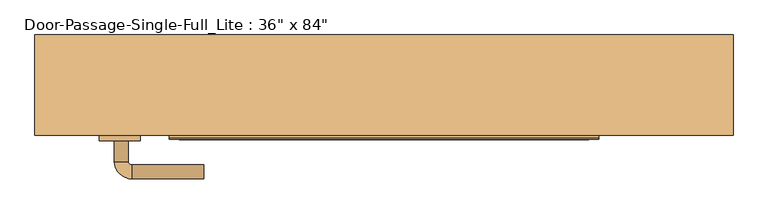
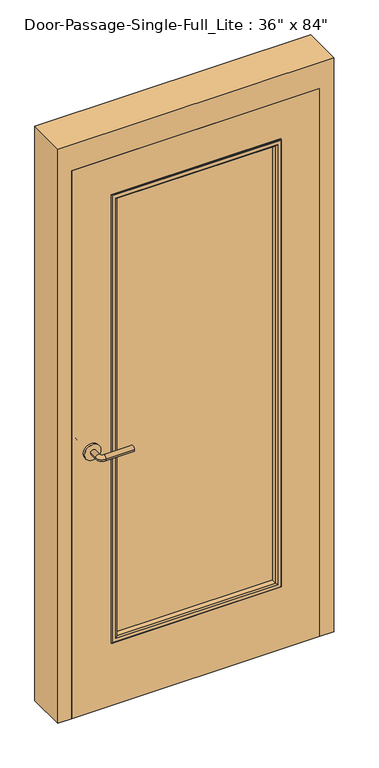
"""IFC4 building model written with IfcOpenShell, lengths in millimetres: door geometry."""

from ifc_helpers import new_model, si_unit, point, frame, frame_2d, origin, place, context, project, spatial, polyline, circle_curve, ellipse_curve, trimmed, segment, composite_curve, outline, extrude, faceted_brep, source, transform, mapped, element, save
from ifc_brep_helpers import plane_surface, cylinder_surface, revolved_surface, advanced_brep


def door_5fc50167(model_context):
    return source(origin(), model_context, "Body", "SolidModel", [
        advanced_brep(
        [(-392.190625, 9.5875, 1016.0), (-372.190625, 9.5875, 1016.0), (-392.190625, 39.5875, 1016.0), (-372.190625, 39.5875, 1016.0), (-367.190625, 44.5875, 1016.0), (-367.190625, 64.5875, 1016.0), (-262.190625, 64.5875, 1016.0), (-262.190625, 44.5875, 1016.0)],
        [
            (0, 1, circle_curve(frame((-382.190625, 9.5875, 1016.0), z_axis=(0.0, -1.0, 0.0), x_axis=(1.0, 0.0, 0.0)), 10.0)),
            (1, 0, circle_curve(frame((-382.190625, 9.5875, 1016.0), z_axis=(0.0, -1.0, 0.0), x_axis=(1.0, 0.0, 0.0)), 10.0)),
            (0, 2),
            (2, 3, circle_curve(frame((-382.190625, 39.5875, 1016.0), z_axis=(0.0, -1.0, 0.0), x_axis=(1.0, 0.0, 0.0)), 10.0)),
            (3, 1),
            (3, 2, circle_curve(frame((-382.190625, 39.5875, 1016.0), z_axis=(0.0, -1.0, 0.0), x_axis=(1.0, 0.0, 0.0)), 10.0)),
            (4, 3, circle_curve(frame((-367.190625, 39.5875, 1016.0), z_axis=(0.0, 0.0, 1.0), x_axis=(-1.0, 0.0, 0.0)), 5.0)),
            (2, 5, circle_curve(frame((-367.190625, 39.5875, 1016.0), z_axis=(0.0, 0.0, -1.0), x_axis=(-1.0, 0.0, 0.0)), 25.0)),
            (5, 4, circle_curve(frame((-367.190625, 54.5875, 1016.0), z_axis=(-1.0, 0.0, 0.0), x_axis=(0.0, -1.0, 0.0)), 10.0)),
            (4, 5, circle_curve(frame((-367.190625, 54.5875, 1016.0), z_axis=(-1.0, 0.0, 0.0), x_axis=(0.0, -1.0, 0.0)), 10.0)),
            (6, 7, circle_curve(frame((-262.190625, 54.5875, 1016.0), z_axis=(1.0, 0.0, 0.0), x_axis=(0.0, -1.0, 0.0)), 10.0)),
            (7, 6, circle_curve(frame((-262.190625, 54.5875, 1016.0), z_axis=(1.0, 0.0, 0.0), x_axis=(0.0, -1.0, 0.0)), 10.0)),
            (5, 6),
            (7, 4),
        ],
        [
            plane_surface(frame((-382.190625, 9.5875, 1016.0), z_axis=(0.0, -1.0, 0.0), x_axis=(0.0, 0.0, 1.0))),
            cylinder_surface(frame((-382.190625, 9.5875, 1016.0), z_axis=(0.0, -1.0, 0.0), x_axis=(1.0, 0.0, 0.0)), 10.0),
            revolved_surface(trimmed(ellipse_curve(frame((-382.190625, 39.5875, 1016.0), z_axis=(0.0, -1.0, 0.0), x_axis=(1.0, 0.0, 0.0)), 10.0, 10.0), [point((-392.190625, 39.5875, 1016.0))], [point((-372.190625, 39.5875, 1016.0))], True, "CARTESIAN"), (-367.190625, 39.5875, 1016.0), (0.0, 0.0, -1.0)),
            revolved_surface(trimmed(ellipse_curve(frame((-382.190625, 39.5875, 1016.0), z_axis=(0.0, -1.0, 0.0), x_axis=(1.0, 0.0, 0.0)), 10.0, 10.0), [point((-372.190625, 39.5875, 1016.0))], [point((-392.190625, 39.5875, 1016.0))], True, "CARTESIAN"), (-367.190625, 39.5875, 1016.0), (0.0, 0.0, -1.0)),
            plane_surface(frame((-262.190625, 54.5875, 1016.0), z_axis=(1.0, 0.0, 0.0), x_axis=(0.0, 0.0, 1.0))),
            cylinder_surface(frame((-367.190625, 54.5875, 1016.0), z_axis=(-1.0, 0.0, 0.0), x_axis=(0.0, -1.0, 0.0)), 10.0),
        ],
        [
            (0, [[1, 2]]),
            (1, [[-1, 3, 4, 5]]),
            (1, [[-2, -5, 6, -3]]),
            (2, [[7, -4, 8, 9]]),
            (3, [[-8, -6, -7, 10]]),
            (4, [[11, 12]]),
            (5, [[-9, 13, -12, 14]]),
            (5, [[-10, -14, -11, -13]]),
        ],
    ),
        extrude(outline(composite_curve([segment(trimmed(circle_curve(frame_2d((1016.0, -384.690625)), 30.0), [point((1016.0, -414.690625))], [point((1016.0, -354.690625))], False, "CARTESIAN"), True, "CONTINUOUS"), segment(trimmed(circle_curve(frame_2d((1016.0, -384.690625)), 30.0), [point((1016.0, -354.690625))], [point((1016.0, -414.690625))], False, "CARTESIAN"), True, "CONTINUOUS")], self_intersect=False)), frame((0.0, 1.5875, 0.0), z_axis=(0.0, 1.0, 0.0), x_axis=(0.0, 0.0, 1.0)), (0.0, 0.0, 1.0), 8.0),
        advanced_brep(
        [(-392.190625, -50.8625, 1016.0), (-372.190625, -50.8625, 1016.0), (-372.190625, -80.8625, 1016.0), (-392.190625, -80.8625, 1016.0), (-367.190625, -85.8625, 1016.0), (-367.190625, -105.8625, 1016.0), (-262.190625, -105.8625, 1016.0), (-262.190625, -85.8625, 1016.0)],
        [
            (0, 1, circle_curve(frame((-382.190625, -50.8625, 1016.0), z_axis=(0.0, 1.0, 0.0), x_axis=(1.0, 0.0, 0.0)), 10.0)),
            (1, 0, circle_curve(frame((-382.190625, -50.8625, 1016.0), z_axis=(0.0, 1.0, 0.0), x_axis=(1.0, 0.0, 0.0)), 10.0)),
            (1, 2),
            (2, 3, circle_curve(frame((-382.190625, -80.8625, 1016.0), z_axis=(0.0, 1.0, 0.0), x_axis=(1.0, 0.0, 0.0)), 10.0)),
            (3, 0),
            (3, 2, circle_curve(frame((-382.190625, -80.8625, 1016.0), z_axis=(0.0, 1.0, 0.0), x_axis=(1.0, 0.0, 0.0)), 10.0)),
            (4, 5, circle_curve(frame((-367.190625, -95.8625, 1016.0), z_axis=(-1.0, 0.0, 0.0), x_axis=(0.0, 1.0, 0.0)), 10.0)),
            (5, 3, circle_curve(frame((-367.190625, -80.8625, 1016.0), z_axis=(0.0, 0.0, -1.0), x_axis=(-1.0, 0.0, 0.0)), 25.0)),
            (2, 4, circle_curve(frame((-367.190625, -80.8625, 1016.0), z_axis=(0.0, 0.0, 1.0), x_axis=(-1.0, 0.0, 0.0)), 5.0)),
            (5, 4, circle_curve(frame((-367.190625, -95.8625, 1016.0), z_axis=(-1.0, 0.0, 0.0), x_axis=(0.0, 1.0, 0.0)), 10.0)),
            (6, 7, circle_curve(frame((-262.190625, -95.8625, 1016.0), z_axis=(1.0, 0.0, 0.0), x_axis=(0.0, 1.0, 0.0)), 10.0)),
            (7, 6, circle_curve(frame((-262.190625, -95.8625, 1016.0), z_axis=(1.0, 0.0, 0.0), x_axis=(0.0, 1.0, 0.0)), 10.0)),
            (4, 7),
            (6, 5),
        ],
        [
            plane_surface(frame((-382.190625, -50.8625, 1016.0), z_axis=(0.0, 1.0, 0.0), x_axis=(0.0, 0.0, 1.0))),
            cylinder_surface(frame((-382.190625, -50.8625, 1016.0), z_axis=(0.0, 1.0, 0.0), x_axis=(1.0, 0.0, 0.0)), 10.0),
            revolved_surface(trimmed(ellipse_curve(frame((-382.190625, -80.8625, 1016.0), z_axis=(0.0, -1.0, 0.0), x_axis=(1.0, 0.0, 0.0)), 10.0, 10.0), [point((-392.190625, -80.8625, 1016.0))], [point((-372.190625, -80.8625, 1016.0))], True, "CARTESIAN"), (-367.190625, -80.8625, 1016.0), (0.0, 0.0, -1.0)),
            revolved_surface(trimmed(ellipse_curve(frame((-382.190625, -80.8625, 1016.0), z_axis=(0.0, -1.0, 0.0), x_axis=(1.0, 0.0, 0.0)), 10.0, 10.0), [point((-372.190625, -80.8625, 1016.0))], [point((-392.190625, -80.8625, 1016.0))], True, "CARTESIAN"), (-367.190625, -80.8625, 1016.0), (0.0, 0.0, -1.0)),
            plane_surface(frame((-262.190625, -95.8625, 1016.0), z_axis=(1.0, 0.0, 0.0), x_axis=(0.0, 0.0, 1.0))),
            cylinder_surface(frame((-367.190625, -95.8625, 1016.0), z_axis=(-1.0, 0.0, 0.0), x_axis=(0.0, 1.0, 0.0)), 10.0),
        ],
        [
            (0, [[1, 2]]),
            (1, [[3, 4, 5, -2]]),
            (1, [[-5, 6, -3, -1]]),
            (2, [[7, 8, -4, 9]]),
            (3, [[10, -9, -6, -8]]),
            (4, [[11, 12]]),
            (5, [[13, -11, 14, -7]]),
            (5, [[-14, -12, -13, -10]]),
        ],
    ),
        extrude(outline(composite_curve([segment(trimmed(circle_curve(frame_2d((1016.0, -384.690625)), 30.0), [point((1016.0, -414.690625))], [point((1016.0, -354.690625))], False, "CARTESIAN"), True, "CONTINUOUS"), segment(trimmed(circle_curve(frame_2d((1016.0, -384.690625)), 30.0), [point((1016.0, -354.690625))], [point((1016.0, -414.690625))], False, "CARTESIAN"), True, "CONTINUOUS")], self_intersect=False)), frame((0.0, -50.8625, 0.0), z_axis=(0.0, 1.0, 0.0), x_axis=(0.0, 0.0, 1.0)), (0.0, 0.0, 1.0), 8.0),
        extrude(outline(polyline([(304.8, -17.4625), (304.8, -23.8125), (-304.8, -23.8125), (-304.8, -17.4625), (304.8, -17.4625)])), frame((0.0, 0.0, 254.0), z_axis=(0.0, 0.0, 1.0), x_axis=(1.0, 0.0, 0.0)), (0.0, 0.0, 1.0), 1727.2),
        faceted_brep([(457.2, 6.35, 0.0), (441.325, 6.35, 0.0), (441.325, 53.975, 0.0), (457.2, 53.975, 0.0), (457.2, 103.1875, 0.0), (508.0, 103.1875, 0.0), (508.0, -42.8625, 0.0), (457.2, -42.8625, 0.0), (457.2, -42.8625, 2133.6), (457.2, 6.35, 2133.6), (508.0, -42.8625, 2235.2), (-508.0, -42.8625, 2235.2), (-508.0, -42.8625, 0.0), (-457.2, -42.8625, 0.0), (-457.2, -42.8625, 2133.6), (508.0, 103.1875, 2235.2), (457.2, 103.1875, 2133.6), (-457.2, 103.1875, 2133.6), (-457.2, 103.1875, 0.0), (-508.0, 103.1875, 0.0), (-508.0, 103.1875, 2235.2), (457.2, 53.975, 2133.6), (441.325, 53.975, 2117.725), (-441.325, 53.975, 2117.725), (-441.325, 53.975, 0.0), (-457.2, 53.975, 0.0), (-457.2, 53.975, 2133.6), (441.325, 6.35, 2117.725), (-457.2, 6.35, 2133.6), (-457.2, 6.35, 0.0), (-441.325, 6.35, 0.0), (-441.325, 6.35, 2117.725)], [[[0, 1, 2, 3, 4, 5, 6, 7]], [[7, 8, 9, 0]], [[6, 10, 11, 12, 13, 14, 8, 7]], [[5, 15, 10, 6]], [[4, 16, 17, 18, 19, 20, 15, 5]], [[3, 21, 16, 4]], [[2, 22, 23, 24, 25, 26, 21, 3]], [[1, 27, 22, 2]], [[0, 9, 28, 29, 30, 31, 27, 1]], [[8, 14, 28, 9]], [[16, 21, 26, 17]], [[22, 27, 31, 23]], [[12, 19, 18, 25, 24, 30, 29, 13]], [[13, 29, 28, 14]], [[11, 20, 19, 12]], [[17, 26, 25, 18]], [[23, 31, 30, 24]], [[15, 20, 11, 10]]]),
        extrude(outline(polyline([(2133.6, -457.2), (0.0, -457.2), (0.0, 457.2), (2133.6, 457.2), (2133.6, -457.2)]), holes=[polyline([(1981.2, -304.8), (1981.2, 304.8), (254.0, 304.8), (254.0, -304.8), (1981.2, -304.8)])]), frame((0.0, -42.8625, 0.0), z_axis=(0.0, 1.0, 0.0), x_axis=(0.0, 0.0, 1.0)), (0.0, 0.0, 1.0), 44.45),
        advanced_brep(
        [(-304.8, -23.8125, 1981.2), (-304.8, -23.8125, 254.0), (-304.8, -42.8625, 254.0), (-304.8, -42.8625, 1981.2), (-292.8, -43.8625, 1969.2), (-292.8, -43.8625, 266.0), (-292.8, -23.8125, 266.0), (-292.8, -23.8125, 1969.2), (-297.8, -48.8625, 1974.2), (-297.8, -48.8625, 261.0), (-312.8, -46.8625, 1989.2), (-312.8, -46.8625, 246.0), (-310.8, -48.8625, 248.0), (-310.8, -48.8625, 1987.2), (-312.8, -42.8625, 1989.2), (-312.8, -42.8625, 246.0), (304.8, -23.8125, 254.0), (304.8, -42.8625, 254.0), (292.8, -43.8625, 266.0), (292.8, -23.8125, 266.0), (297.8, -48.8625, 261.0), (312.8, -46.8625, 246.0), (310.8, -48.8625, 248.0), (312.8, -42.8625, 246.0), (304.8, -23.8125, 1981.2), (304.8, -42.8625, 1981.2), (292.8, -43.8625, 1969.2), (292.8, -23.8125, 1969.2), (297.8, -48.8625, 1974.2), (312.8, -46.8625, 1989.2), (310.8, -48.8625, 1987.2), (312.8, -42.8625, 1989.2)],
        [
            (0, 1),
            (1, 2),
            (2, 3),
            (3, 0),
            (4, 5),
            (5, 6),
            (6, 7),
            (7, 4),
            (8, 9),
            (9, 5, ellipse_curve(frame((-297.8, -43.8625, 261.0), z_axis=(-0.7071067811865475, 0.0, 0.7071067811865475), x_axis=(0.7071067811865474, 0.0, 0.7071067811865476)), 7.0710678, 5.0)),
            (4, 8, ellipse_curve(frame((-297.8, -43.8625, 1974.2), z_axis=(-0.7071067811865475, 0.0, -0.7071067811865475), x_axis=(-0.7071067811865474, 0.0, 0.7071067811865476)), 7.0710678, 5.0)),
            (10, 11),
            (11, 12, ellipse_curve(frame((-310.8, -46.8625, 248.0), z_axis=(-0.7071067811865475, 0.0, 0.7071067811865475), x_axis=(0.7071067811865474, 0.0, 0.7071067811865476)), 2.8284271, 2.0)),
            (12, 13),
            (13, 10, ellipse_curve(frame((-310.8, -46.8625, 1987.2), z_axis=(-0.7071067811865475, 0.0, -0.7071067811865475), x_axis=(-0.7071067811865474, 0.0, 0.7071067811865476)), 2.8284271, 2.0)),
            (14, 15),
            (15, 11),
            (10, 14),
            (1, 16),
            (16, 17),
            (17, 2),
            (5, 18),
            (18, 19),
            (19, 6),
            (9, 20),
            (20, 18, ellipse_curve(frame((297.8, -43.8625, 261.0), z_axis=(-0.7071067811865475, 0.0, -0.7071067811865475), x_axis=(-0.7071067811865476, 0.0, 0.7071067811865474)), 7.0710678, 5.0)),
            (11, 21),
            (21, 22, ellipse_curve(frame((310.8, -46.8625, 248.0), z_axis=(-0.7071067811865475, 0.0, -0.7071067811865475), x_axis=(-0.7071067811865476, 0.0, 0.7071067811865474)), 2.8284271, 2.0)),
            (22, 12),
            (15, 23),
            (23, 21),
            (16, 24),
            (24, 25),
            (25, 17),
            (18, 26),
            (26, 27),
            (27, 19),
            (20, 28),
            (28, 26, ellipse_curve(frame((297.8, -43.8625, 1974.2), z_axis=(0.7071067811865475, 0.0, -0.7071067811865475), x_axis=(-0.7071067811865474, 0.0, -0.7071067811865476)), 7.0710678, 5.0)),
            (21, 29),
            (29, 30, ellipse_curve(frame((310.8, -46.8625, 1987.2), z_axis=(0.7071067811865475, 0.0, -0.7071067811865475), x_axis=(-0.7071067811865474, 0.0, -0.7071067811865476)), 2.8284271, 2.0)),
            (30, 22),
            (23, 31),
            (31, 29),
            (14, 31),
            (25, 3),
            (24, 0),
            (27, 7),
            (26, 4),
            (28, 8),
            (30, 13),
            (29, 10),
        ],
        [
            plane_surface(frame((-304.8, -42.8625, 1981.2), z_axis=(-1.0, 0.0, 0.0), x_axis=(0.0, 0.0, -1.0))),
            plane_surface(frame((-292.8, -23.8125, 1969.2), z_axis=(1.0, 0.0, 0.0), x_axis=(0.0, 0.0, -1.0))),
            cylinder_surface(frame((-297.8, -43.8625, 1981.2), z_axis=(0.0, 0.0, 1.0), x_axis=(-1.0, 0.0, 0.0)), 5.0),
            cylinder_surface(frame((-310.8, -46.8625, 1981.2), z_axis=(0.0, 0.0, 1.0), x_axis=(-1.0, 0.0, 0.0)), 2.0),
            plane_surface(frame((-312.8, -46.8625, 1989.2), z_axis=(-1.0, 0.0, 0.0), x_axis=(0.0, 0.0, -1.0))),
            plane_surface(frame((-304.8, -42.8625, 254.0), z_axis=(0.0, 0.0, -1.0), x_axis=(1.0, 0.0, 0.0))),
            plane_surface(frame((-292.8, -23.8125, 266.0), z_axis=(0.0, 0.0, 1.0), x_axis=(1.0, 0.0, 0.0))),
            cylinder_surface(frame((-304.8, -43.8625, 261.0), z_axis=(-1.0, 0.0, 0.0), x_axis=(0.0, 0.0, -1.0)), 5.0),
            cylinder_surface(frame((-304.8, -46.8625, 248.0), z_axis=(-1.0, 0.0, 0.0), x_axis=(0.0, 0.0, -1.0)), 2.0),
            plane_surface(frame((-312.8, -46.8625, 246.0), z_axis=(0.0, 0.0, -1.0), x_axis=(1.0, 0.0, 0.0))),
            plane_surface(frame((304.8, -42.8625, 254.0), z_axis=(1.0, 0.0, 0.0), x_axis=(0.0, 0.0, 1.0))),
            plane_surface(frame((292.8, -23.8125, 266.0), z_axis=(-1.0, 0.0, 0.0), x_axis=(0.0, 0.0, 1.0))),
            cylinder_surface(frame((297.8, -43.8625, 254.0), z_axis=(0.0, 0.0, -1.0), x_axis=(1.0, 0.0, 0.0)), 5.0),
            cylinder_surface(frame((310.8, -46.8625, 254.0), z_axis=(0.0, 0.0, -1.0), x_axis=(1.0, 0.0, 0.0)), 2.0),
            plane_surface(frame((312.8, -46.8625, 246.0), z_axis=(1.0, 0.0, 0.0), x_axis=(0.0, 0.0, 1.0))),
            plane_surface(frame((312.8, -42.8625, 1989.2), z_axis=(0.0, 1.0, 0.0), x_axis=(-1.0, 0.0, 0.0))),
            plane_surface(frame((304.8, -42.8625, 1981.2), z_axis=(0.0, 0.0, 1.0), x_axis=(-1.0, 0.0, 0.0))),
            plane_surface(frame((304.8, -23.8125, 1981.2), z_axis=(0.0, 1.0, 0.0), x_axis=(-1.0, 0.0, 0.0))),
            plane_surface(frame((292.8, -23.8125, 1969.2), z_axis=(0.0, 0.0, -1.0), x_axis=(-1.0, 0.0, 0.0))),
            cylinder_surface(frame((304.8, -43.8625, 1974.2), z_axis=(1.0, 0.0, 0.0), x_axis=(0.0, 0.0, 1.0)), 5.0),
            plane_surface(frame((297.8, -48.8625, 1974.2), z_axis=(0.0, -1.0, 0.0), x_axis=(-1.0, 0.0, 0.0))),
            cylinder_surface(frame((304.8, -46.8625, 1987.2), z_axis=(1.0, 0.0, 0.0), x_axis=(0.0, 0.0, 1.0)), 2.0),
            plane_surface(frame((312.8, -46.8625, 1989.2), z_axis=(0.0, 0.0, 1.0), x_axis=(-1.0, 0.0, 0.0))),
        ],
        [
            (0, [[1, 2, 3, 4]]),
            (1, [[5, 6, 7, 8]]),
            (2, [[9, 10, -5, 11]]),
            (3, [[12, 13, 14, 15]]),
            (4, [[16, 17, -12, 18]]),
            (5, [[19, 20, 21, -2]]),
            (6, [[22, 23, 24, -6]]),
            (7, [[25, 26, -22, -10]]),
            (8, [[27, 28, 29, -13]]),
            (9, [[30, 31, -27, -17]]),
            (10, [[32, 33, 34, -20]]),
            (11, [[35, 36, 37, -23]]),
            (12, [[38, 39, -35, -26]]),
            (13, [[40, 41, 42, -28]]),
            (14, [[43, 44, -40, -31]]),
            (15, [[-16, 45, -43, -30], [-3, -21, -34, 46]]),
            (16, [[47, -4, -46, -33]]),
            (17, [[-1, -47, -32, -19], [-7, -24, -37, 48]]),
            (18, [[49, -8, -48, -36]]),
            (19, [[50, -11, -49, -39]]),
            (20, [[-14, -29, -42, 51], [-9, -50, -38, -25]]),
            (21, [[52, -15, -51, -41]]),
            (22, [[-45, -18, -52, -44]]),
        ],
    ),
        advanced_brep(
        [(-304.8, -17.4625, 254.0), (-304.8, -17.4625, 1981.2), (-304.8, 1.5875, 1981.2), (-304.8, 1.5875, 254.0), (-292.8, 2.5875, 266.0), (-292.8, 2.5875, 1969.2), (-292.8, -17.4625, 1969.2), (-292.8, -17.4625, 266.0), (-297.8, 7.5875, 261.0), (-297.8, 7.5875, 1974.2), (-312.8, 5.5875, 246.0), (-312.8, 5.5875, 1989.2), (-310.8, 7.5875, 1987.2), (-310.8, 7.5875, 248.0), (-312.8, 1.5875, 246.0), (-312.8, 1.5875, 1989.2), (304.8, -17.4625, 1981.2), (304.8, 1.5875, 1981.2), (292.8, 2.5875, 1969.2), (292.8, -17.4625, 1969.2), (297.8, 7.5875, 1974.2), (312.8, 5.5875, 1989.2), (310.8, 7.5875, 1987.2), (312.8, 1.5875, 1989.2), (304.8, -17.4625, 254.0), (304.8, 1.5875, 254.0), (292.8, 2.5875, 266.0), (292.8, -17.4625, 266.0), (297.8, 7.5875, 261.0), (312.8, 5.5875, 246.0), (310.8, 7.5875, 248.0), (312.8, 1.5875, 246.0)],
        [
            (0, 1),
            (1, 2),
            (2, 3),
            (3, 0),
            (4, 5),
            (5, 6),
            (6, 7),
            (7, 4),
            (8, 9),
            (9, 5, ellipse_curve(frame((-297.8, 2.5875, 1974.2), z_axis=(-0.7071067811865475, 0.0, -0.7071067811865475), x_axis=(0.7071067811865474, 0.0, -0.7071067811865476)), 7.0710678, 5.0)),
            (4, 8, ellipse_curve(frame((-297.8, 2.5875, 261.0), z_axis=(-0.7071067811865475, 0.0, 0.7071067811865475), x_axis=(-0.7071067811865474, 0.0, -0.7071067811865476)), 7.0710678, 5.0)),
            (10, 11),
            (11, 12, ellipse_curve(frame((-310.8, 5.5875, 1987.2), z_axis=(-0.7071067811865475, 0.0, -0.7071067811865475), x_axis=(0.7071067811865474, 0.0, -0.7071067811865476)), 2.8284271, 2.0)),
            (12, 13),
            (13, 10, ellipse_curve(frame((-310.8, 5.5875, 248.0), z_axis=(-0.7071067811865475, 0.0, 0.7071067811865475), x_axis=(-0.7071067811865474, 0.0, -0.7071067811865476)), 2.8284271, 2.0)),
            (14, 15),
            (15, 11),
            (10, 14),
            (1, 16),
            (16, 17),
            (17, 2),
            (5, 18),
            (18, 19),
            (19, 6),
            (9, 20),
            (20, 18, ellipse_curve(frame((297.8, 2.5875, 1974.2), z_axis=(-0.7071067811865475, 0.0, 0.7071067811865475), x_axis=(-0.7071067811865476, 0.0, -0.7071067811865474)), 7.0710678, 5.0)),
            (11, 21),
            (21, 22, ellipse_curve(frame((310.8, 5.5875, 1987.2), z_axis=(-0.7071067811865475, 0.0, 0.7071067811865475), x_axis=(-0.7071067811865476, 0.0, -0.7071067811865474)), 2.8284271, 2.0)),
            (22, 12),
            (15, 23),
            (23, 21),
            (16, 24),
            (24, 25),
            (25, 17),
            (18, 26),
            (26, 27),
            (27, 19),
            (20, 28),
            (28, 26, ellipse_curve(frame((297.8, 2.5875, 261.0), z_axis=(0.7071067811865475, 0.0, 0.7071067811865475), x_axis=(-0.7071067811865474, 0.0, 0.7071067811865476)), 7.0710678, 5.0)),
            (21, 29),
            (29, 30, ellipse_curve(frame((310.8, 5.5875, 248.0), z_axis=(0.7071067811865475, 0.0, 0.7071067811865475), x_axis=(-0.7071067811865474, 0.0, 0.7071067811865476)), 2.8284271, 2.0)),
            (30, 22),
            (23, 31),
            (31, 29),
            (14, 31),
            (25, 3),
            (24, 0),
            (27, 7),
            (26, 4),
            (28, 8),
            (30, 13),
            (29, 10),
        ],
        [
            plane_surface(frame((-304.8, 1.5875, 254.0), z_axis=(-1.0, 0.0, 0.0), x_axis=(0.0, 0.0, 1.0))),
            plane_surface(frame((-292.8, -17.4625, 266.0), z_axis=(1.0, 0.0, 0.0), x_axis=(0.0, 0.0, 1.0))),
            cylinder_surface(frame((-297.8, 2.5875, 254.0), z_axis=(0.0, 0.0, -1.0), x_axis=(-1.0, 0.0, 0.0)), 5.0),
            cylinder_surface(frame((-310.8, 5.5875, 254.0), z_axis=(0.0, 0.0, -1.0), x_axis=(-1.0, 0.0, 0.0)), 2.0),
            plane_surface(frame((-312.8, 5.5875, 246.0), z_axis=(-1.0, 0.0, 0.0), x_axis=(0.0, 0.0, 1.0))),
            plane_surface(frame((-304.8, 1.5875, 1981.2), z_axis=(0.0, 0.0, 1.0), x_axis=(1.0, 0.0, 0.0))),
            plane_surface(frame((-292.8, -17.4625, 1969.2), z_axis=(0.0, 0.0, -1.0), x_axis=(1.0, 0.0, 0.0))),
            cylinder_surface(frame((-304.8, 2.5875, 1974.2), z_axis=(-1.0, 0.0, 0.0), x_axis=(0.0, 0.0, 1.0)), 5.0),
            cylinder_surface(frame((-304.8, 5.5875, 1987.2), z_axis=(-1.0, 0.0, 0.0), x_axis=(0.0, 0.0, 1.0)), 2.0),
            plane_surface(frame((-312.8, 5.5875, 1989.2), z_axis=(0.0, 0.0, 1.0), x_axis=(1.0, 0.0, 0.0))),
            plane_surface(frame((304.8, 1.5875, 1981.2), z_axis=(1.0, 0.0, 0.0), x_axis=(0.0, 0.0, -1.0))),
            plane_surface(frame((292.8, -17.4625, 1969.2), z_axis=(-1.0, 0.0, 0.0), x_axis=(0.0, 0.0, -1.0))),
            cylinder_surface(frame((297.8, 2.5875, 1981.2), z_axis=(0.0, 0.0, 1.0), x_axis=(1.0, 0.0, 0.0)), 5.0),
            cylinder_surface(frame((310.8, 5.5875, 1981.2), z_axis=(0.0, 0.0, 1.0), x_axis=(1.0, 0.0, 0.0)), 2.0),
            plane_surface(frame((312.8, 5.5875, 1989.2), z_axis=(1.0, 0.0, 0.0), x_axis=(0.0, 0.0, -1.0))),
            plane_surface(frame((312.8, 1.5875, 246.0), z_axis=(0.0, -1.0, 0.0), x_axis=(-1.0, 0.0, 0.0))),
            plane_surface(frame((304.8, 1.5875, 254.0), z_axis=(0.0, 0.0, -1.0), x_axis=(-1.0, 0.0, 0.0))),
            plane_surface(frame((304.8, -17.4625, 254.0), z_axis=(0.0, -1.0, 0.0), x_axis=(-1.0, 0.0, 0.0))),
            plane_surface(frame((292.8, -17.4625, 266.0), z_axis=(0.0, 0.0, 1.0), x_axis=(-1.0, 0.0, 0.0))),
            cylinder_surface(frame((304.8, 2.5875, 261.0), z_axis=(1.0, 0.0, 0.0), x_axis=(0.0, 0.0, -1.0)), 5.0),
            plane_surface(frame((297.8, 7.5875, 261.0), z_axis=(0.0, 1.0, 0.0), x_axis=(-1.0, 0.0, 0.0))),
            cylinder_surface(frame((304.8, 5.5875, 248.0), z_axis=(1.0, 0.0, 0.0), x_axis=(0.0, 0.0, -1.0)), 2.0),
            plane_surface(frame((312.8, 5.5875, 246.0), z_axis=(0.0, 0.0, -1.0), x_axis=(-1.0, 0.0, 0.0))),
        ],
        [
            (0, [[1, 2, 3, 4]]),
            (1, [[5, 6, 7, 8]]),
            (2, [[9, 10, -5, 11]]),
            (3, [[12, 13, 14, 15]]),
            (4, [[16, 17, -12, 18]]),
            (5, [[19, 20, 21, -2]]),
            (6, [[22, 23, 24, -6]]),
            (7, [[25, 26, -22, -10]]),
            (8, [[27, 28, 29, -13]]),
            (9, [[30, 31, -27, -17]]),
            (10, [[32, 33, 34, -20]]),
            (11, [[35, 36, 37, -23]]),
            (12, [[38, 39, -35, -26]]),
            (13, [[40, 41, 42, -28]]),
            (14, [[43, 44, -40, -31]]),
            (15, [[-16, 45, -43, -30], [-3, -21, -34, 46]]),
            (16, [[47, -4, -46, -33]]),
            (17, [[-1, -47, -32, -19], [-7, -24, -37, 48]]),
            (18, [[49, -8, -48, -36]]),
            (19, [[50, -11, -49, -39]]),
            (20, [[-14, -29, -42, 51], [-9, -50, -38, -25]]),
            (21, [[52, -15, -51, -41]]),
            (22, [[-45, -18, -52, -44]]),
        ],
    ),
    ])


if __name__ == "__main__":
    model = new_model("IFC4")
    model_context = context("Model", 3, world=origin())
    ifc_project = project(units=[si_unit("LENGTHUNIT", "METRE", prefix="MILLI")], contexts=[model_context])
    site = spatial("IfcSite", under=ifc_project)
    building = spatial("IfcBuilding", under=site)
    placement = place(None, origin())
    door_shape = door_5fc50167(model_context)
    element("IfcDoor", 1, ObjectType="Door-Passage-Single-Full_Lite : 36\" x 84\"", at=placement, inside=building, context=model_context, shape_type="MappedRepresentation", body=[
        mapped(door_shape, transform((0.0, 0.0, 0.0), x_axis=(1.0, 0.0, 0.0), y_axis=(0.0, 1.0, 0.0), z_axis=(0.0, 0.0, 1.0))),
    ])
    save(model, "model.ifc")

# Revit data of these elements
# Type "Door-Passage-Single-Full_Lite : 36\" x 84\""
#   Type Mark = "52"
#   Assembly Code = "B2030100"
#   Analytic Construction = "Wooden"
#   Thickness = 0' - 1 3/4"
#   Thermal Resistance (R) = 2.5876 (h·ft²·°F)/BTU
#   Swing Angle [instance default] = 90.00°
#   Strike Height = 3' - 4"
#   Rough Width [instance default] = 3' - 4"
#   Rough Height [instance default] = 7' - 4"
#   MF Opening Height [instance default] = 0' - 4"
#   MF Opening Width [instance default] = 0' - 4"
#   Inset Calculate [instance default] = 0' - 4"
#   Masonry Inset [instance default] = 0' - 1"
#   Height = 7' - 0"
#   Width = 3' - 0"
#   Heat Transfer Coefficient (U) = 0.3865 BTU/(h·ft²·°F)
#   Masonry Frame Depth = 0' - 5 3/4"
#   Masonry Frame [instance default] = yes
#   Function = 1
#   Dry Wall Frame [instance default] = no
#   Panel Material = Wood - Birch
#   Glazing = Glass
#   Glass Stop Material = Metal - Paint Finish - Grey
#   Frame Material = Metal - Paint Finish - Grey
#   Door Handle Material = Aluminum
#   Visual Light Transmittance = 0
#   Solar Heat Gain Coefficient = 0
#   Wall Closure = (empty or 0)
# Element 1 (IfcDoor, "Door-Passage-Single-Full_Lite : 36\" x 84\"")
#   Materials on its faces: "Metal - Paint Finish - Grey", "Aluminum", "Wood - Birch", "Glass"
# Materials
#   "Wood - Birch": class "Wood", colour RGB 166 116 52, transparency 0, Cost = 0
#   "Glass": class "Glass", colour RGB 0 128 192, transparency 0.75, Description = "Soda Lime Glass", Cost = 0
#   "Metal - Paint Finish - Grey": class "Paint", colour RGB 104 104 104, transparency 0, Cost = 0
#   "Aluminum": class "Metal", colour RGB 247 247 247, transparency 0, Description = "Aluminum 6061", Cost = 0
